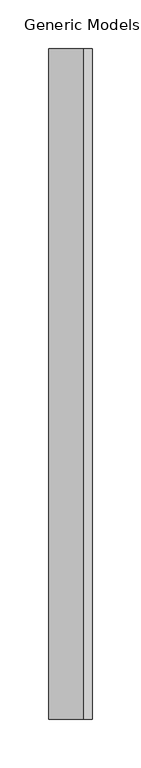
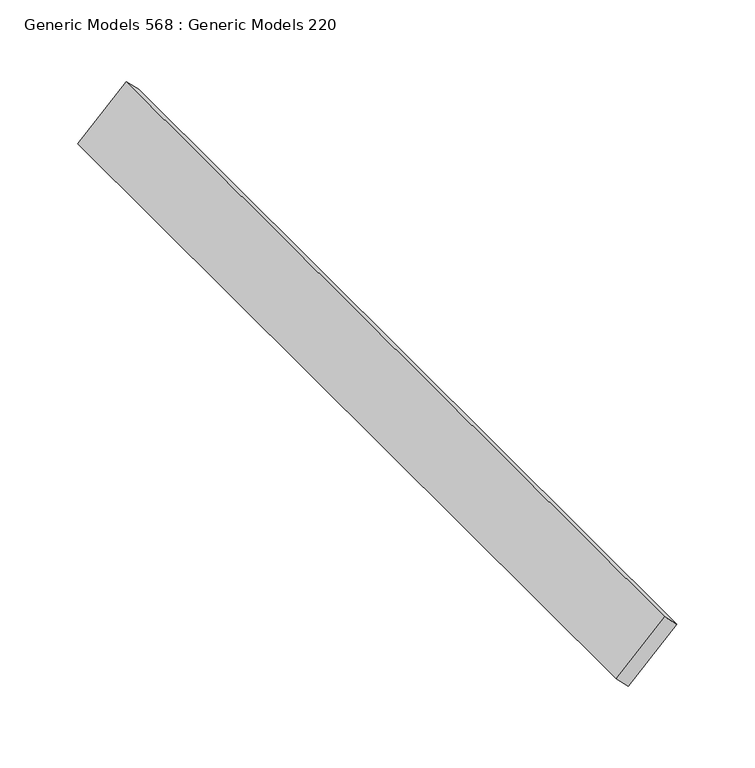
"""IFC4 building model written with IfcOpenShell, lengths in millimetres: proxy geometry, Generic Models 568 : Generic Models 220."""

from ifc_helpers import new_model, si_unit, frame, origin, place, context, project, spatial, polyline, outline, extrude, source, transform, mapped, element, save


def generic_models_568_generic_models_220_3dfde852(model_context):
    return source(origin(), model_context, "Body", "SweptSolid", [
        extrude(outline(polyline([(0.0, -12.7000001), (0.0, 0.0), (690.8142348, 0.0), (690.8142348, -12.7000001), (0.0, -12.7000001)])), frame((7841.3059863, 4539.4872686, 124112.6399101), z_axis=(0.7071067811868034, 0.0, 0.7071067811862918), x_axis=(0.0, -1.0, 0.0)), (0.0, 0.0, 1.0), 50.8),
    ])


if __name__ == "__main__":
    model = new_model("IFC4")
    model_context = context("Model", 3, world=origin())
    ifc_project = project(units=[si_unit("LENGTHUNIT", "METRE", prefix="MILLI")], contexts=[model_context])
    site = spatial("IfcSite", under=ifc_project)
    building = spatial("IfcBuilding", under=site)
    placement = place(None, origin())
    generic_models_568_generic_models_220_shape = generic_models_568_generic_models_220_3dfde852(model_context)
    element("IfcBuildingElementProxy", 1, Name="Generic Models 568 : Generic Models 220", ObjectType="Generic Models 568 : Generic Models 220", at=placement, inside=building, context=model_context, shape_type="MappedRepresentation", body=[
        mapped(generic_models_568_generic_models_220_shape, transform((0.0, 0.0, 0.0), x_axis=(1.0, 0.0, 0.0), y_axis=(0.0, 1.0, 0.0), z_axis=(0.0, 0.0, 1.0))),
    ])
    save(model, "model.ifc")

# Revit data of these elements
# Element 1 (IfcBuildingElementProxy, "Generic Models 568 : Generic Models 220")
#   Materials on its faces: "_WOOD TONE ALUMINUM EXTRUSION SLAT BY KNOTWOOD"
# Materials
#   "_WOOD TONE ALUMINUM EXTRUSION SLAT BY KNOTWOOD": class "Generic", colour RGB 177 130 114, transparency 0, Cost = 0
